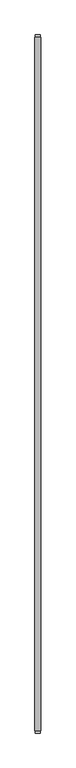
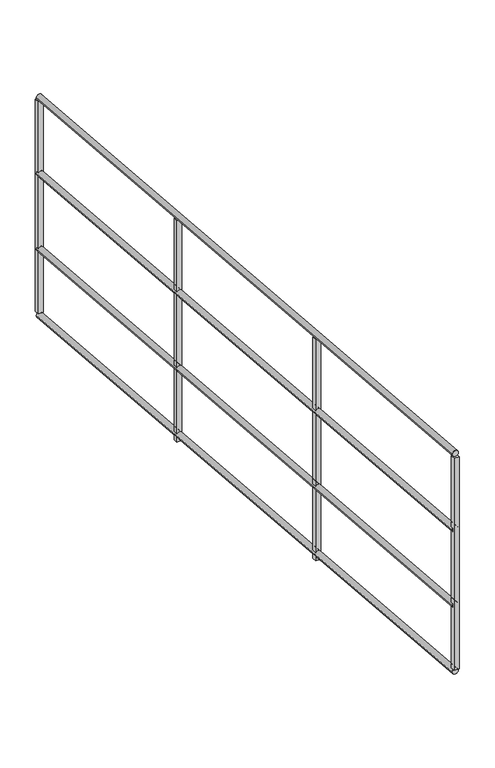
"""IFC4 building model written with IfcOpenShell, lengths in millimetres: railing geometry."""

from ifc_helpers import new_model, si_unit, frame, origin, place, context, project, spatial, polyline, ellipse_curve, outline, extrude, source, transform, mapped, element, save
from ifc_brep_helpers import plane_surface, cylinder_surface, advanced_brep


def railing_86a8b08b(model_context):
    return source(origin(), model_context, "Body", "SolidModel", [
        advanced_brep(
        [(22390.0, 22999.5208589, 1034.9098701), (22360.0, 22999.5208589, 1034.9098701), (22390.0, 19399.5208589, 1334.9098701), (22360.0, 19399.5208589, 1334.9098701)],
        [
            (0, 1, ellipse_curve(frame((22375.0, 22999.5208589, 1034.9098701), z_axis=(0.0, 1.0, 0.0), x_axis=(0.0, 0.0, -1.0)), 15.0519932, 15.0)),
            (1, 0, ellipse_curve(frame((22375.0, 22999.5208589, 1034.9098701), z_axis=(0.0, 1.0, 0.0), x_axis=(0.0, 0.0, -1.0)), 15.0519932, 15.0)),
            (2, 3, ellipse_curve(frame((22375.0, 19399.5208589, 1334.9098701), z_axis=(0.0, -1.0, 0.0), x_axis=(0.0, 0.0, -1.0)), 15.0519932, 15.0)),
            (3, 2, ellipse_curve(frame((22375.0, 19399.5208589, 1334.9098701), z_axis=(0.0, -1.0, 0.0), x_axis=(0.0, 0.0, -1.0)), 15.0519932, 15.0)),
            (0, 2),
            (3, 1),
        ],
        [
            plane_surface(frame((22375.0, 22999.5208589, 1049.9618634), z_axis=(0.0, 1.0, 0.0), x_axis=(0.0, 0.0, -1.0))),
            plane_surface(frame((22375.0, 19399.5208589, 1349.9618634), z_axis=(0.0, -1.0, 0.0), x_axis=(0.0, 0.0, -1.0))),
            cylinder_surface(frame((22375.0, 22998.2751767, 1035.013677), z_axis=(0.0, 0.9965457582448797, -0.08304547985373989), x_axis=(-1.0, 0.0, 0.0)), 15.0),
        ],
        [
            (0, [[1, 2]]),
            (1, [[3, 4]]),
            (2, [[-1, 5, -4, 6]]),
            (2, [[-2, -6, -3, -5]]),
        ],
    ),
        advanced_brep(
        [(22390.0, 22999.5208589, 634.9098701), (22360.0, 22999.5208589, 634.9098701), (22390.0, 19399.5208589, 934.9098701), (22360.0, 19399.5208589, 934.9098701)],
        [
            (0, 1, ellipse_curve(frame((22375.0, 22999.5208589, 634.9098701), z_axis=(0.0, 1.0, 0.0), x_axis=(0.0, 0.0, -1.0)), 15.0519932, 15.0)),
            (1, 0, ellipse_curve(frame((22375.0, 22999.5208589, 634.9098701), z_axis=(0.0, 1.0, 0.0), x_axis=(0.0, 0.0, -1.0)), 15.0519932, 15.0)),
            (2, 3, ellipse_curve(frame((22375.0, 19399.5208589, 934.9098701), z_axis=(0.0, -1.0, 0.0), x_axis=(0.0, 0.0, -1.0)), 15.0519932, 15.0)),
            (3, 2, ellipse_curve(frame((22375.0, 19399.5208589, 934.9098701), z_axis=(0.0, -1.0, 0.0), x_axis=(0.0, 0.0, -1.0)), 15.0519932, 15.0)),
            (0, 2),
            (3, 1),
        ],
        [
            plane_surface(frame((22375.0, 22999.5208589, 649.9618634), z_axis=(0.0, 1.0, 0.0), x_axis=(0.0, 0.0, -1.0))),
            plane_surface(frame((22375.0, 19399.5208589, 949.9618634), z_axis=(0.0, -1.0, 0.0), x_axis=(0.0, 0.0, -1.0))),
            cylinder_surface(frame((22375.0, 22998.2751767, 635.013677), z_axis=(0.0, 0.9965457582448797, -0.08304547985373992), x_axis=(-1.0, 0.0, 0.0)), 15.0),
        ],
        [
            (0, [[1, 2]]),
            (1, [[3, 4]]),
            (2, [[-1, 5, -4, 6]]),
            (2, [[-2, -6, -3, -5]]),
        ],
    ),
        advanced_brep(
        [(22390.0, 22999.5208589, 234.9098701), (22360.0, 22999.5208589, 234.9098701), (22390.0, 19399.5208589, 534.9098701), (22360.0, 19399.5208589, 534.9098701)],
        [
            (0, 1, ellipse_curve(frame((22375.0, 22999.5208589, 234.9098701), z_axis=(0.0, 1.0, 0.0), x_axis=(0.0, 0.0, -1.0)), 15.0519932, 15.0)),
            (1, 0, ellipse_curve(frame((22375.0, 22999.5208589, 234.9098701), z_axis=(0.0, 1.0, 0.0), x_axis=(0.0, 0.0, -1.0)), 15.0519932, 15.0)),
            (2, 3, ellipse_curve(frame((22375.0, 19399.5208589, 534.9098701), z_axis=(0.0, -1.0, 0.0), x_axis=(0.0, 0.0, -1.0)), 15.0519932, 15.0)),
            (3, 2, ellipse_curve(frame((22375.0, 19399.5208589, 534.9098701), z_axis=(0.0, -1.0, 0.0), x_axis=(0.0, 0.0, -1.0)), 15.0519932, 15.0)),
            (0, 2),
            (3, 1),
        ],
        [
            plane_surface(frame((22375.0, 22999.5208589, 249.9618634), z_axis=(0.0, 1.0, 0.0), x_axis=(0.0, 0.0, -1.0))),
            plane_surface(frame((22375.0, 19399.5208589, 549.9618634), z_axis=(0.0, -1.0, 0.0), x_axis=(0.0, 0.0, -1.0))),
            cylinder_surface(frame((22375.0, 22998.2751767, 235.013677), z_axis=(0.0, 0.9965457582448797, -0.08304547985373992), x_axis=(-1.0, 0.0, 0.0)), 15.0),
        ],
        [
            (0, [[1, 2]]),
            (1, [[3, 4]]),
            (2, [[-1, 5, -4, 6]]),
            (2, [[-2, -6, -3, -5]]),
        ],
    ),
        advanced_brep(
        [(22390.0, 22999.5208589, -115.0901299), (22360.0, 22999.5208589, -115.0901299), (22390.0, 19399.5208589, 184.9098701), (22360.0, 19399.5208589, 184.9098701)],
        [
            (0, 1, ellipse_curve(frame((22375.0, 22999.5208589, -115.0901299), z_axis=(0.0, 1.0, 0.0), x_axis=(0.0, 0.0, -1.0)), 15.0519932, 15.0)),
            (1, 0, ellipse_curve(frame((22375.0, 22999.5208589, -115.0901299), z_axis=(0.0, 1.0, 0.0), x_axis=(0.0, 0.0, -1.0)), 15.0519932, 15.0)),
            (2, 3, ellipse_curve(frame((22375.0, 19399.5208589, 184.9098701), z_axis=(0.0, -1.0, 0.0), x_axis=(0.0, 0.0, -1.0)), 15.0519932, 15.0)),
            (3, 2, ellipse_curve(frame((22375.0, 19399.5208589, 184.9098701), z_axis=(0.0, -1.0, 0.0), x_axis=(0.0, 0.0, -1.0)), 15.0519932, 15.0)),
            (0, 2),
            (3, 1),
        ],
        [
            plane_surface(frame((22375.0, 22999.5208589, -100.0381366), z_axis=(0.0, 1.0, 0.0), x_axis=(0.0, 0.0, -1.0))),
            plane_surface(frame((22375.0, 19399.5208589, 199.9618634), z_axis=(0.0, -1.0, 0.0), x_axis=(0.0, 0.0, -1.0))),
            cylinder_surface(frame((22375.0, 22998.2751767, -114.986323), z_axis=(0.0, 0.9965457582448797, -0.08304547985373992), x_axis=(-1.0, 0.0, 0.0)), 15.0),
        ],
        [
            (0, [[1, 2]]),
            (1, [[3, 4]]),
            (2, [[-1, 5, -4, 6]]),
            (2, [[-2, -6, -3, -5]]),
        ],
    ),
        extrude(outline(polyline([(20612.0208589, 1218.8162103), (20612.0208589, 48.9201967), (20587.0208589, 51.00353), (20587.0208589, 1220.8995436), (20612.0208589, 1218.8162103)])), frame((22362.5, 0.0, 0.0), z_axis=(1.0, 0.0, 0.0), x_axis=(0.0, 1.0, 0.0)), (0.0, 0.0, 1.0), 25.0),
        extrude(outline(polyline([(21812.0208589, 1118.8162103), (21812.0208589, -51.0798033), (21787.0208589, -48.99647), (21787.0208589, 1120.8995436), (21812.0208589, 1118.8162103)])), frame((22362.5, 0.0, 0.0), z_axis=(1.0, 0.0, 0.0), x_axis=(0.0, 1.0, 0.0)), (0.0, 0.0, 1.0), 25.0),
        extrude(outline(polyline([(19412.0208589, 1318.8162103), (19412.0208589, 198.9201967), (19387.0208589, 201.00353), (19387.0208589, 1320.8995436), (19412.0208589, 1318.8162103)])), frame((22362.5, 0.0, 0.0), z_axis=(1.0, 0.0, 0.0), x_axis=(0.0, 1.0, 0.0)), (0.0, 0.0, 1.0), 25.0),
        extrude(outline(polyline([(23012.0208589, 1018.8162103), (23012.0208589, -101.0798033), (22987.0208589, -98.99647), (22987.0208589, 1020.8995436), (23012.0208589, 1018.8162103)])), frame((22362.5, 0.0, 0.0), z_axis=(1.0, 0.0, 0.0), x_axis=(0.0, 1.0, 0.0)), (0.0, 0.0, 1.0), 25.0),
    ])


if __name__ == "__main__":
    model = new_model("IFC4")
    model_context = context("Model", 3, world=origin())
    ifc_project = project(units=[si_unit("LENGTHUNIT", "METRE", prefix="MILLI")], contexts=[model_context])
    site = spatial("IfcSite", under=ifc_project)
    building = spatial("IfcBuilding", under=site)
    placement = place(None, origin())
    railing_shape = railing_86a8b08b(model_context)
    element("IfcRailing", 1, at=placement, inside=building, context=model_context, shape_type="MappedRepresentation", body=[
        mapped(railing_shape, transform((0.0, 0.0, 0.0), x_axis=(1.0, 0.0, 0.0), y_axis=(0.0, 1.0, 0.0), z_axis=(0.0, 0.0, 1.0))),
    ])
    save(model, "model.ifc")
